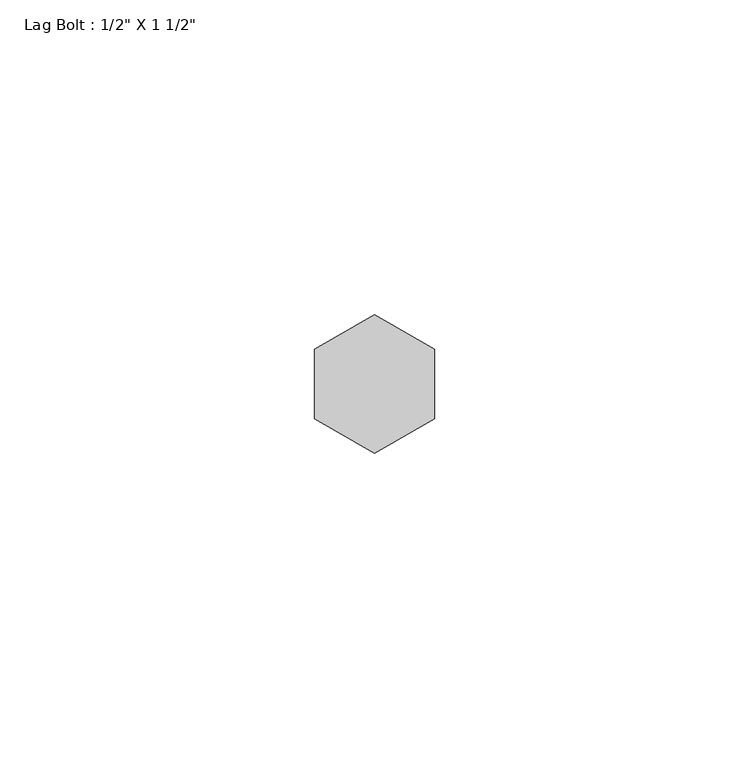
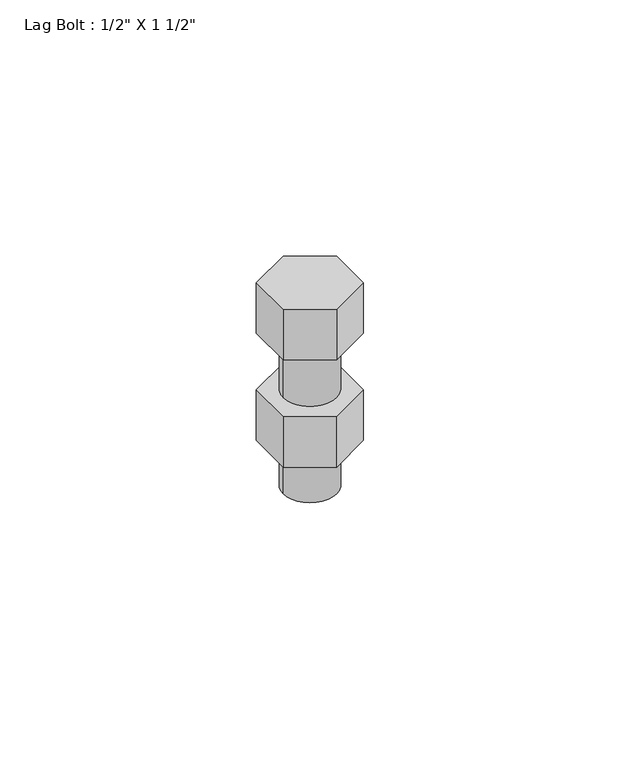
"""IFC4 building model written with IfcOpenShell, lengths in millimetres: proxy geometry."""

from ifc_helpers import new_model, si_unit, point, frame, origin, origin_with_axes, origin_2d, place, context, project, spatial, polyline, circle_curve, trimmed, segment, composite_curve, outline, extrude, source, transform, mapped, element, save


def proxy_ced08073(model_context):
    return source(origin(), model_context, "Body", "SweptSolid", [
        extrude(outline(polyline([(-9.525, -5.4992613), (-9.525, 5.4992613), (0.0, 10.9985226), (9.525, 5.4992613), (9.525, -5.4992613), (0.0, -10.9985226), (-9.525, -5.4992613)])), frame((0.0, 0.0, -26.8882812), z_axis=(0.0, 0.0, 1.0), x_axis=(1.0, 0.0, 0.0)), (0.0, 0.0, 1.0), 12.7),
        extrude(outline(polyline([(-9.525, 5.4992613), (0.0, 10.9985226), (9.525, 5.4992613), (9.525, -5.4992613), (0.0, -10.9985226), (-9.525, -5.4992613), (-9.525, 5.4992613)])), origin_with_axes(), (0.0, 0.0, 1.0), 12.7),
        extrude(outline(composite_curve([segment(trimmed(circle_curve(origin_2d(), 6.35), [point((-6.35, 0.0))], [point((6.35, 0.0))], False, "CARTESIAN"), True, "CONTINUOUS"), segment(trimmed(circle_curve(origin_2d(), 6.35), [point((6.35, 0.0))], [point((-6.35, 0.0))], False, "CARTESIAN"), True, "CONTINUOUS")], self_intersect=False)), frame((0.0, 0.0, -38.1), z_axis=(0.0, 0.0, 1.0), x_axis=(1.0, 0.0, 0.0)), (0.0, 0.0, 1.0), 38.1),
    ])


if __name__ == "__main__":
    model = new_model("IFC4")
    model_context = context("Model", 3, world=origin())
    ifc_project = project(units=[si_unit("LENGTHUNIT", "METRE", prefix="MILLI")], contexts=[model_context])
    site = spatial("IfcSite", under=ifc_project)
    building = spatial("IfcBuilding", under=site)
    placement = place(None, origin())
    proxy_shape = proxy_ced08073(model_context)
    element("IfcBuildingElementProxy", 1, Name="Lag Bolt : 1/2\" X 1 1/2\"", ObjectType="Lag Bolt : 1/2\" X 1 1/2\"", at=placement, inside=building, context=model_context, shape_type="MappedRepresentation", body=[
        mapped(proxy_shape, transform((0.0, 0.0, 0.0), x_axis=(1.0, 0.0, 0.0), y_axis=(0.0, 1.0, 0.0), z_axis=(0.0, 0.0, 1.0))),
    ])
    save(model, "model.ifc")

# Revit data of these elements
# Type "Lag Bolt : 1/2\" X 1 1/2\""
#   Thickness_of_Substrate [instance default] = 0' - 1"
#   Side = 0' - 0 111/256"
#   Radius = 0' - 0 1/4"
#   Length = 0' - 1 1/2"
#   Head Size = 0' - 0 3/4"
#   Head Radius = 0' - 0 3/8"
#   Head Height = 0' - 0 1/2"
#   Diameter = 0' - 0 1/2"
#   Default Elevation = 4' - 0"
#   Nut_Visibility [instance default] = yes
#   Bolt Material (Size) [instance default] = 1/2" X 5" LAG BOLT (THRU BOLT IF PLATE ON OPP. SIDE OF STRUCT MEMBER)
# Element 1 (IfcBuildingElementProxy, "Lag Bolt : 1/2\" X 1 1/2\"")
#   Thickness_of_Substrate = 0' - 0 143/256"
#   Bolt Material (Size) = THRU-BOLT OR LAG BOLT
#   Materials on its faces: "THRU-BOLT OR LAG BOLT"
# Materials
#   "1/2\" X 5\" LAG BOLT (THRU BOLT IF PLATE ON OPP. SIDE OF STRUCT MEMBER)": class "Generic", colour RGB 120 120 120, transparency 0, Cost = 0
#   "THRU-BOLT OR LAG BOLT": class "Generic", colour RGB 120 120 120, transparency 0, Cost = 0
